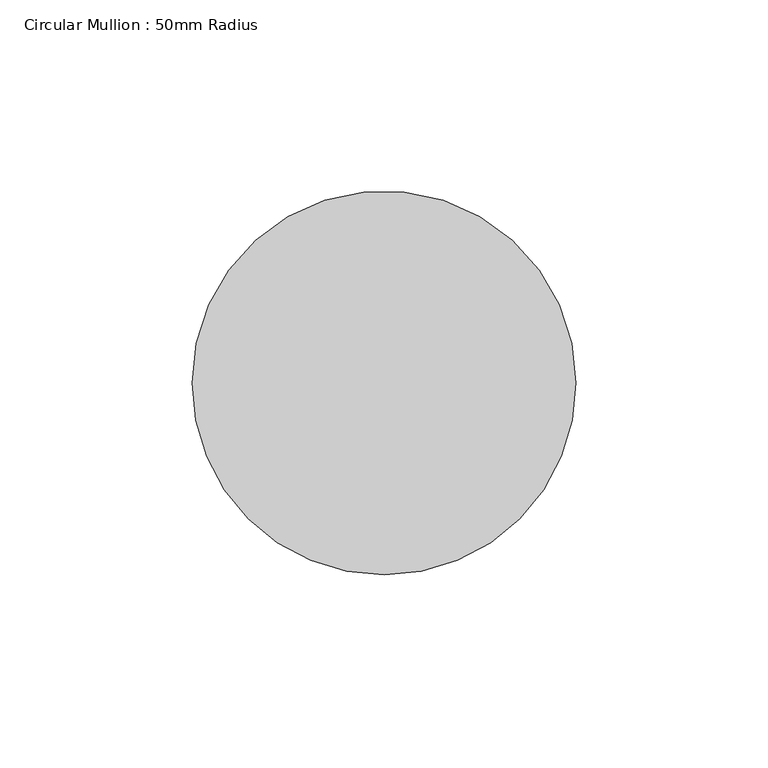
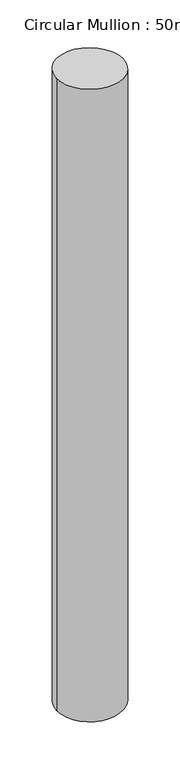
"""IFC4 building model written with IfcOpenShell, lengths in millimetres: member geometry, Circular Mullion : 50mm Radius."""

from ifc_helpers import new_model, si_unit, frame, origin, place, context, project, spatial, ellipse_curve, source, transform, mapped, element, save
from ifc_brep_helpers import plane_surface, cylinder_surface, advanced_brep


def circular_mullion_50mm_radius_86e7b0e0(model_context):
    return source(origin(), model_context, "Body", "AdvancedBrep", [
        advanced_brep(
        [(-100.0, 0.0, 2.1144719), (0.0, 0.0, 0.0), (0.0, 0.0, -1010.7417029), (-100.0, 0.0, -1012.8980844)],
        [
            (0, 1, ellipse_curve(frame((-50.0, 0.0, 1.057236), z_axis=(-0.02113471657319806, -0.02234261995256583, -0.9995269536580922), x_axis=(-0.6868714457152116, -0.7261279144545549, 0.03075498188869349)), 50.0236635, 50.0)),
            (1, 2),
            (2, 3, ellipse_curve(frame((-50.0, 0.0, -1011.8198937), z_axis=(-0.021553206096955706, -0.022785027228340176, 0.999508029903285), x_axis=(0.6868584413767611, 0.7261141668846799, 0.0313639627415568)), 50.0246106, 50.0)),
            (3, 0),
            (1, 0, ellipse_curve(frame((-50.0, 0.0, 1.057236), z_axis=(-0.02113471657319806, -0.02234261995256583, -0.9995269536580922), x_axis=(-0.6868714457152116, -0.7261279144545549, 0.03075498188869349)), 50.0236635, 50.0)),
            (3, 2, ellipse_curve(frame((-50.0, 0.0, -1011.8198937), z_axis=(-0.021553206096955706, -0.022785027228340176, 0.999508029903285), x_axis=(0.6868584413767611, 0.7261141668846799, 0.0313639627415568)), 50.0246106, 50.0)),
        ],
        [
            cylinder_surface(frame((-50.0, 0.0, 0.0), z_axis=(0.0, 0.0, 1.0), x_axis=(1.0, 0.0, 0.0)), 50.0),
            plane_surface(frame((-221.4285343, 209.4574998, 0.0), z_axis=(0.02113471657319806, 0.02234261995256583, 0.9995269536580922), x_axis=(0.6868714457152115, 0.7261279144545546, -0.03075498188869903))),
            plane_surface(frame((-221.4285343, 209.4574998, -1010.7417029), z_axis=(0.021553206096955706, 0.022785027228340176, -0.999508029903285), x_axis=(0.6868584413767611, 0.7261141668846797, 0.0313639627415614))),
        ],
        [
            (0, [[1, 2, 3, 4]]),
            (0, [[5, -4, 6, -2]]),
            (1, [[-1, -5]]),
            (2, [[-6, -3]]),
        ],
    ),
    ])


if __name__ == "__main__":
    model = new_model("IFC4")
    model_context = context("Model", 3, world=origin())
    ifc_project = project(units=[si_unit("LENGTHUNIT", "METRE", prefix="MILLI")], contexts=[model_context])
    site = spatial("IfcSite", under=ifc_project)
    building = spatial("IfcBuilding", under=site)
    placement = place(None, origin())
    circular_mullion_50mm_radius_shape = circular_mullion_50mm_radius_86e7b0e0(model_context)
    element("IfcMember", 1, ObjectType="Circular Mullion : 50mm Radius", at=placement, inside=building, context=model_context, shape_type="MappedRepresentation", body=[
        mapped(circular_mullion_50mm_radius_shape, transform((0.0, 0.0, 0.0), x_axis=(1.0, 0.0, 0.0), y_axis=(0.0, 1.0, 0.0), z_axis=(0.0, 0.0, 1.0))),
    ])
    save(model, "model.ifc")

# Revit data of these elements
# Type "Circular Mullion : 50mm Radius"
#   built-in parameter 1007350 = 0.164042 (stored number, unit not read)
# Element 1 (IfcMember, "Circular Mullion : 50mm Radius")
#   Materials on its faces: "Aluminium"
# Materials
#   "Aluminium": class "Metal", colour RGB 247 247 247, transparency 0, Description = "Aluminium 6061", Cost = 0
